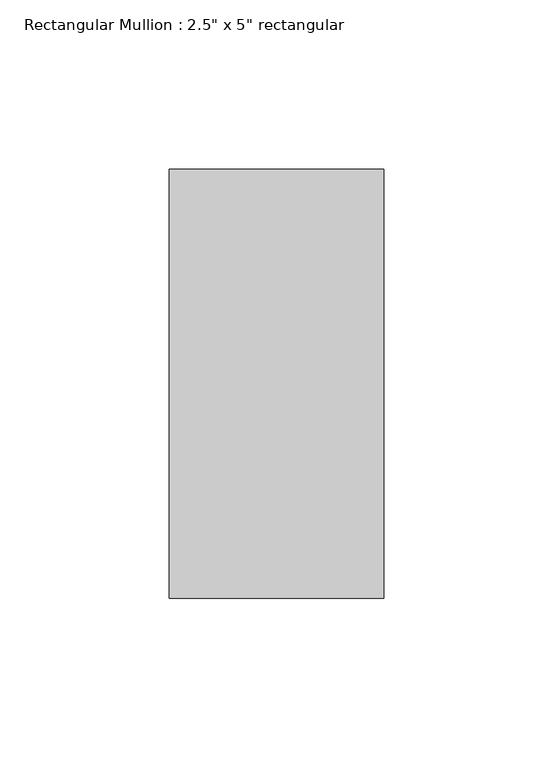
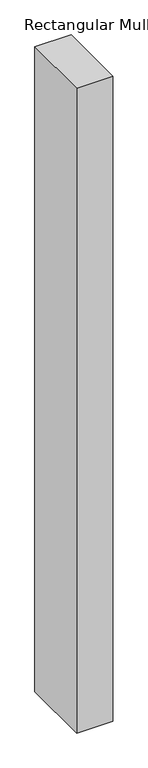
"""IFC4 building model written with IfcOpenShell, lengths in millimetres: member geometry."""

from ifc_helpers import new_model, si_unit, frame, origin, place, context, project, spatial, polyline, outline, extrude, source, transform, mapped, element, save


def member_e9ca7dfe(model_context):
    return source(origin(), model_context, "Body", "SweptSolid", [
        extrude(outline(polyline([(0.0, 63.5), (0.0, -63.5), (-63.5, -63.5), (-63.5, 63.5), (0.0, 63.5)])), frame((0.0, 0.0, -1198.0333333), z_axis=(0.0, 0.0, 1.0), x_axis=(1.0, 0.0, 0.0)), (0.0, 0.0, 1.0), 1198.0333333),
    ])


if __name__ == "__main__":
    model = new_model("IFC4")
    model_context = context("Model", 3, world=origin())
    ifc_project = project(units=[si_unit("LENGTHUNIT", "METRE", prefix="MILLI")], contexts=[model_context])
    site = spatial("IfcSite", under=ifc_project)
    building = spatial("IfcBuilding", under=site)
    placement = place(None, origin())
    member_shape = member_e9ca7dfe(model_context)
    element("IfcMember", 1, ObjectType="Rectangular Mullion : 2.5\" x 5\" rectangular", at=placement, inside=building, context=model_context, shape_type="MappedRepresentation", body=[
        mapped(member_shape, transform((0.0, 0.0, 0.0), x_axis=(1.0, 0.0, 0.0), y_axis=(0.0, 1.0, 0.0), z_axis=(0.0, 0.0, 1.0))),
    ])
    save(model, "model.ifc")

# Revit data of these elements
# Type "Rectangular Mullion : 2.5\" x 5\" rectangular"
#   built-in parameter 1007304 = 0.416667 (stored number, unit not read)
#   built-in parameter 1007301 = 0.104167 (stored number, unit not read)
#   built-in parameter 1007300 = 0.104167 (stored number, unit not read)
